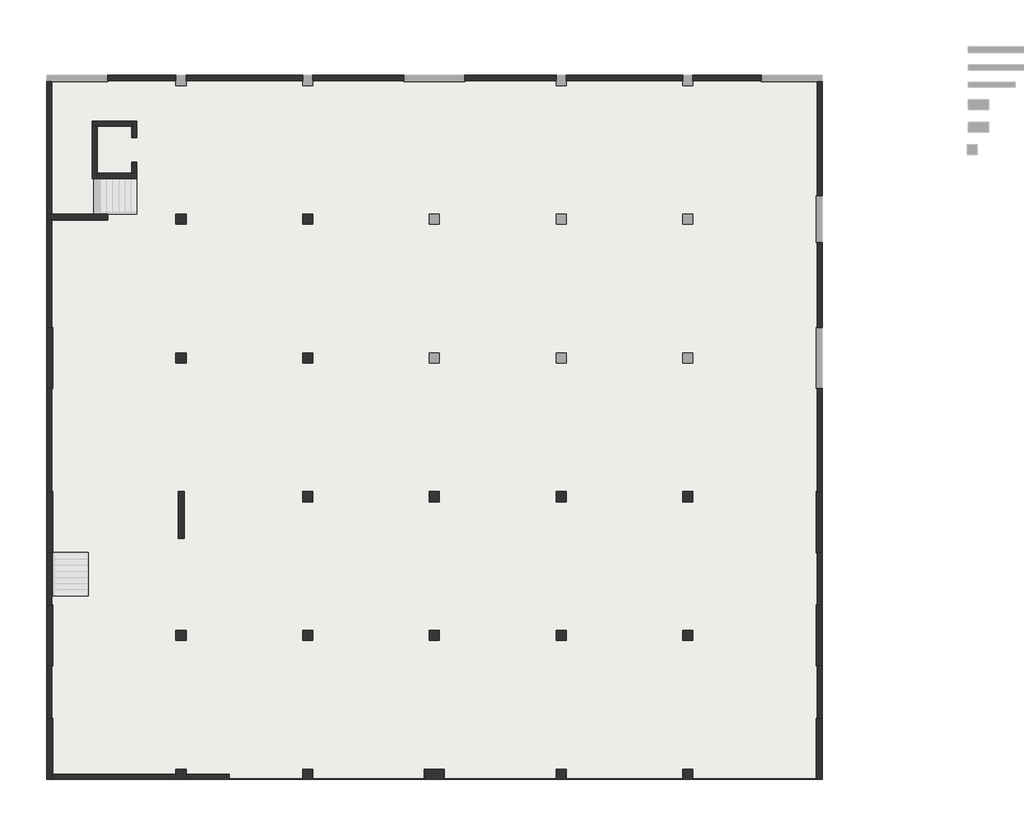
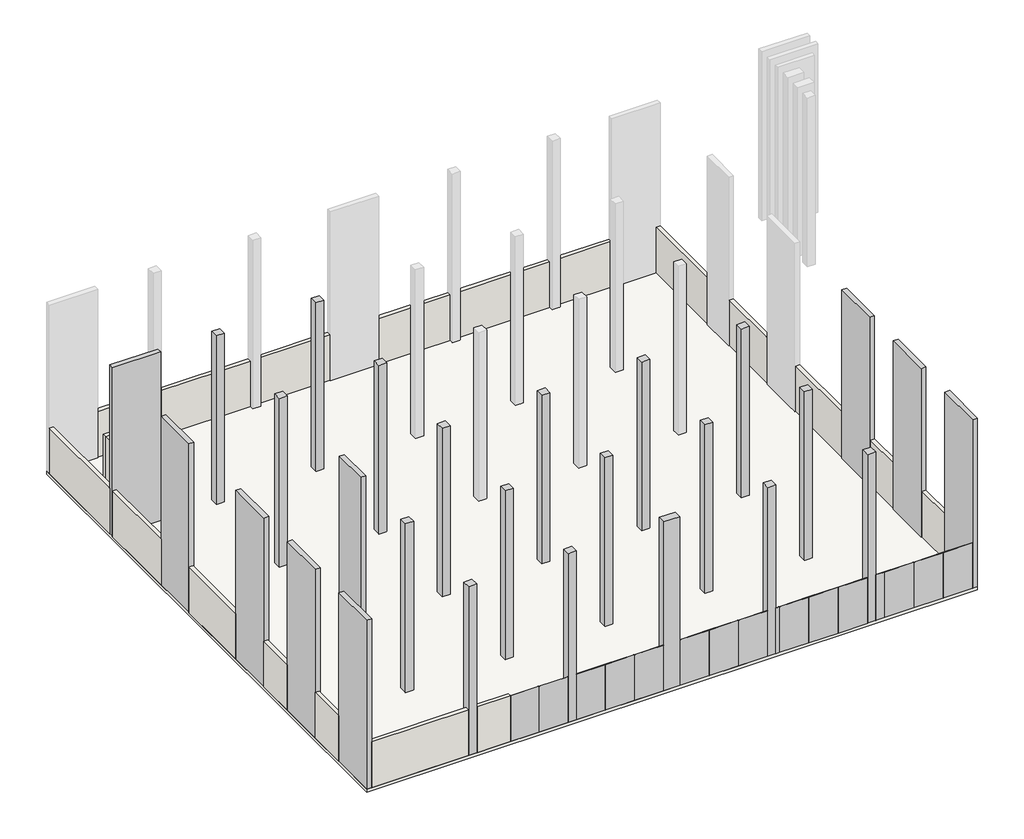
# One storey, part 1 of 2: 27 columns, 23 walls, 16 plates, 1 slab.
"""IFC4 building model written with IfcOpenShell, lengths in millimetres."""

import ifcopenshell
import ifcopenshell.guid

model = None  # the IFC model being written
_history = None  # IfcOwnerHistory: only IFC2X3 demands one
_inside = {}  # id of a spatial element -> (the spatial element, [elements in it])
_under = {}  # id of a project, library or spatial element -> (it, [spatial elements below it])
_declared = {}  # id of a project -> (the project, [libraries it declares])
_typed = {}  # id of a type object -> (the type object, [elements of that type])
_made_of = {}  # id of a material, layer set ... -> (it, [elements and type objects made of it])


def new_model(schema):
    """Start an empty IFC model of exactly this schema.

    Asked for "IFC4X3", IfcOpenShell would pick the latest addendum, in which some entities
    have other attributes; the version numbers below select the first issue.
    IFC2X3 requires an IfcOwnerHistory on every rooted entity: one is made here for all.
    """
    global model, _history
    if schema == "IFC4X3":
        model = ifcopenshell.file(schema_version=(4, 3, 0, 0))
    else:
        model = ifcopenshell.file(schema=schema)
    _inside.clear()
    _under.clear()
    _declared.clear()
    _typed.clear()
    _made_of.clear()
    _history = None
    if model.schema == "IFC2X3":
        org = make("IfcOrganization", Name="unknown")
        user = make(
            "IfcPersonAndOrganization",
            ThePerson=make("IfcPerson", FamilyName="unknown"),
            TheOrganization=org,
        )
        app = make(
            "IfcApplication",
            ApplicationDeveloper=org,
            Version="unknown",
            ApplicationFullName="unknown",
            ApplicationIdentifier="unknown",
        )
        _history = make(
            "IfcOwnerHistory",
            OwningUser=user,
            OwningApplication=app,
            ChangeAction="ADDED",
            CreationDate=0,
        )
    return model


def make(cls, **values):
    """One entity of the class cls with the attributes given. An attribute that is None is left unset."""
    return model.create_entity(
        cls, **{name: value for name, value in values.items() if value is not None}
    )


def rooted(cls, **values):
    """An entity with a GlobalId (a new one), such as an element, a storey or a relation."""
    return make(cls, GlobalId=ifcopenshell.guid.new(), OwnerHistory=_history, **values)


def si_unit(unit_type, name, prefix=None):
    """IfcSIUnit, for example si_unit("LENGTHUNIT", "METRE", prefix="MILLI")."""
    return make("IfcSIUnit", UnitType=unit_type, Prefix=prefix, Name=name)


def assignment(units):
    """IfcUnitAssignment: the units of a project."""
    return None if units is None else make("IfcUnitAssignment", Units=units)


def point(xyz):
    """IfcCartesianPoint."""
    return None if xyz is None else make("IfcCartesianPoint", Coordinates=xyz)


def direction(xyz):
    """IfcDirection."""
    return None if xyz is None else make("IfcDirection", DirectionRatios=xyz)


def frame(location, z_axis=None, x_axis=None):
    """IfcAxis2Placement3D, a coordinate frame: its origin and axes. An axis left out is left unset."""
    return make(
        "IfcAxis2Placement3D",
        Location=point(location),
        Axis=direction(z_axis),
        RefDirection=direction(x_axis),
    )


def origin():
    """The frame at (0, 0, 0) with its axes left unset."""
    return frame((0.0, 0.0, 0.0))


def origin_with_axes():
    """The frame at (0, 0, 0) with the z axis (0, 0, 1) and the x axis (1, 0, 0) written out."""
    return frame((0.0, 0.0, 0.0), z_axis=(0.0, 0.0, 1.0), x_axis=(1.0, 0.0, 0.0))


def place(relative_to, where):
    """IfcLocalPlacement: puts the frame where relative to a parent placement (None: the world)."""
    return make(
        "IfcLocalPlacement", PlacementRelTo=relative_to, RelativePlacement=where
    )


def context(
    kind, dimensions, precision=None, world=None, true_north=None, identifier=None
):
    """IfcGeometricRepresentationContext, for example the 3D "Model" context."""
    return make(
        "IfcGeometricRepresentationContext",
        ContextIdentifier=identifier,
        ContextType=kind,
        CoordinateSpaceDimension=dimensions,
        Precision=precision,
        WorldCoordinateSystem=world,
        TrueNorth=true_north,
    )


def project(units=None, contexts=None):
    """IfcProject with its units and contexts."""
    return rooted(
        "IfcProject",
        Name="project",
        RepresentationContexts=contexts,
        UnitsInContext=assignment(units),
    )


def spatial(cls, under=None, at=None, **own):
    """A site, building, storey or space (cls), placed at a placement, below another one or the project."""
    s = rooted(cls, ObjectPlacement=at, **own)
    if under is not None:
        _under.setdefault(under.id(), (under, []))[1].append(s)
    return s


def polyline(points):
    """IfcPolyline through the points."""
    return make("IfcPolyline", Points=[point(p) for p in points])


def outline(outer, holes=None, kind="AREA"):
    """IfcArbitraryClosedProfileDef: a profile drawn as a closed curve; with holes, ...WithVoids."""
    if holes is None:
        return make("IfcArbitraryClosedProfileDef", ProfileType=kind, OuterCurve=outer)
    return make(
        "IfcArbitraryProfileDefWithVoids",
        ProfileType=kind,
        OuterCurve=outer,
        InnerCurves=holes,
    )


def extrude(swept, where, along, depth):
    """IfcExtrudedAreaSolid: the profile swept, set in the frame where, extruded along a direction by depth."""
    return make(
        "IfcExtrudedAreaSolid",
        SweptArea=swept,
        Position=where,
        ExtrudedDirection=direction(along),
        Depth=depth,
    )


def faces_of(points, faces, orient=None, outer=None):
    """IfcFace entities. A face is a list of loops; a loop is a list of indices into points, from 0.

    orient and outer hold one flag for each loop. By default every Orientation is true, the
    first loop of a face is its IfcFaceOuterBound and the others are IfcFaceBound.
    """
    made = []
    for i, loops in enumerate(faces):
        bounds = []
        for j, loop in enumerate(loops):
            is_outer = j == 0 if outer is None else outer[i][j]
            bounds.append(
                make(
                    "IfcFaceOuterBound" if is_outer else "IfcFaceBound",
                    Bound=make("IfcPolyLoop", Polygon=[points[k] for k in loop]),
                    Orientation=True if orient is None else orient[i][j],
                )
            )
        made.append(make("IfcFace", Bounds=bounds))
    return made


def faceted_brep(points, faces, orient=None, outer=None, voids=None):
    """IfcFacetedBrep: a solid bounded by flat faces; with voids (closed shells), ...WithVoids."""
    shared = [point(p) for p in points]
    hull = make("IfcClosedShell", CfsFaces=faces_of(shared, faces, orient, outer))
    if voids is None:
        return make("IfcFacetedBrep", Outer=hull)
    return make(
        "IfcFacetedBrepWithVoids",
        Outer=hull,
        Voids=[
            make(cls, CfsFaces=faces_of(shared, fs, o, b)) for cls, fs, o, b in voids
        ],
    )


def shape(context_of_items, identifier, shape_type, items):
    """IfcShapeRepresentation: the items that make up one representation, for example the "Body"."""
    return make(
        "IfcShapeRepresentation",
        ContextOfItems=context_of_items,
        RepresentationIdentifier=identifier,
        RepresentationType=shape_type,
        Items=items,
    )


def source(mapping_origin, context_of_items, identifier, shape_type, items):
    """IfcRepresentationMap: a shape defined once, which mapped items show again and again."""
    return make(
        "IfcRepresentationMap",
        MappingOrigin=mapping_origin,
        MappedRepresentation=shape(context_of_items, identifier, shape_type, items),
    )


def transform(
    local_origin,
    x_axis=None,
    y_axis=None,
    z_axis=None,
    scale=None,
    scale2=None,
    scale3=None,
    uniform=True,
):
    """IfcCartesianTransformationOperator3D, or its non-uniform kind. x_axis, y_axis, z_axis: its Axis1, 2, 3."""
    if uniform:
        return make(
            "IfcCartesianTransformationOperator3D",
            Axis1=direction(x_axis),
            Axis2=direction(y_axis),
            LocalOrigin=point(local_origin),
            Scale=scale,
            Axis3=direction(z_axis),
        )
    return make(
        "IfcCartesianTransformationOperator3DnonUniform",
        Axis1=direction(x_axis),
        Axis2=direction(y_axis),
        LocalOrigin=point(local_origin),
        Scale=scale,
        Axis3=direction(z_axis),
        Scale2=scale2,
        Scale3=scale3,
    )


def mapped(mapping_source, mapping_target):
    """IfcMappedItem: shows the shape of a source again, moved by a transform."""
    return make(
        "IfcMappedItem", MappingSource=mapping_source, MappingTarget=mapping_target
    )


def made_of(thing, what):
    """Note that an element or type object is made of a material, layer set ...; save() writes the relation."""
    if what is not None:
        _made_of.setdefault(what.id(), (what, []))[1].append(thing)
    return thing


def element(
    cls,
    number,
    at=None,
    inside=None,
    cuts=None,
    type_object=None,
    material=None,
    context=None,
    identifier="Body",
    shape_type=None,
    held_by="IfcProductDefinitionShape",
    body=None,
    shapes=None,
    **own,
):
    """One element of the class cls, such as IfcWall. Its Tag is "e" and its number.

    at: its placement. inside: the storey or other place that contains it. cuts: it is an
    opening in that element (IfcRelVoidsElement). A single representation is given by context,
    identifier, shape_type and body (its items); several are given by shapes. held_by: the class
    of the entity that holds the representations. save() writes the other relations.
    """
    e = rooted(cls, Tag="e%d" % number, ObjectPlacement=at, **own)
    if body is not None:
        shapes = [shape(context, identifier, shape_type, body)]
    if shapes is not None:
        e.Representation = make(held_by, Representations=shapes)
    if inside is not None:
        _inside.setdefault(inside.id(), (inside, []))[1].append(e)
    if cuts is not None:
        rooted(
            "IfcRelVoidsElement", RelatingBuildingElement=cuts, RelatedOpeningElement=e
        )
    if type_object is not None:
        _typed.setdefault(type_object.id(), (type_object, []))[1].append(e)
    return made_of(e, material)


def aggregate(whole, parts):
    """IfcRelAggregates: a whole, such as a stair, and the parts it consists of."""
    return rooted("IfcRelAggregates", RelatingObject=whole, RelatedObjects=parts)


def save(model, path):
    """Write the relations noted so far, then the file.

    IfcRelAggregates (storeys below a building ...), IfcRelContainedInSpatialStructure (elements
    in a storey), IfcRelDefinesByType, IfcRelAssociatesMaterial and IfcRelDeclares: one each for
    every whole, place, type object, material and project.
    """
    for whole, parts in _under.values():
        aggregate(whole, parts)
    for where, things in _inside.values():
        rooted(
            "IfcRelContainedInSpatialStructure",
            RelatedElements=things,
            RelatingStructure=where,
        )
    for kind, things in _typed.values():
        rooted("IfcRelDefinesByType", RelatedObjects=things, RelatingType=kind)
    for what, things in _made_of.values():
        rooted("IfcRelAssociatesMaterial", RelatedObjects=things, RelatingMaterial=what)
    for by, libraries in _declared.values():
        rooted("IfcRelDeclares", RelatingContext=by, RelatedDefinitions=libraries)
    model.write(path)


def m_rectangular_column_100x50_89a3459c(model_context):
    return source(origin(), model_context, "Body", "SweptSolid", [
        extrude(outline(polyline([(500.0, 250.0), (500.0, -250.0), (-500.0, -250.0), (-500.0, 250.0), (500.0, 250.0)])), frame((0.0, 0.0, -3200.0), z_axis=(0.0, 0.0, 1.0), x_axis=(1.0, 0.0, 0.0)), (0.0, 0.0, 1.0), 11100.0),
    ])


def m_rectangular_column_230x30_624f9335(model_context):
    return source(origin(), model_context, "Body", "SweptSolid", [
        extrude(outline(polyline([(1150.0, 150.0), (1150.0, -150.0), (-1150.0, -150.0), (-1150.0, 150.0), (1150.0, 150.0)])), frame((0.0, 0.0, -3200.0), z_axis=(0.0, 0.0, 1.0), x_axis=(1.0, 0.0, 0.0)), (0.0, 0.0, 1.0), 11100.0),
    ])


def m_rectangular_column_300x30_b7aa0491(model_context):
    return source(origin(), model_context, "Body", "SweptSolid", [
        extrude(outline(polyline([(1500.0, 150.0), (1500.0, -150.0), (-1500.0, -150.0), (-1500.0, 150.0), (1500.0, 150.0)])), frame((0.0, 0.0, -3200.0), z_axis=(0.0, 0.0, 1.0), x_axis=(1.0, 0.0, 0.0)), (0.0, 0.0, 1.0), 11100.0),
    ])


def m_rectangular_column_300x30_baf48ca4(model_context):
    return source(origin(), model_context, "Body", "SweptSolid", [
        extrude(outline(polyline([(1500.0, -150.0), (-1500.0, -150.0), (-1500.0, 150.0), (1500.0, 150.0), (1500.0, -150.0)])), frame((0.0, 0.0, -3200.0), z_axis=(0.0, 0.0, 1.0), x_axis=(1.0, 0.0, 0.0)), (0.0, 0.0, 1.0), 11100.0),
    ])


def m_rectangular_column_50x50_3a95f3c9(model_context):
    return source(origin(), model_context, "Body", "SweptSolid", [
        extrude(outline(polyline([(250.0, 250.0), (250.0, -250.0), (-250.0, -250.0), (-250.0, 250.0), (250.0, 250.0)])), frame((0.0, 0.0, -3200.0), z_axis=(0.0, 0.0, 1.0), x_axis=(1.0, 0.0, 0.0)), (0.0, 0.0, 1.0), 11100.0),
    ])


def system_panel_glazed_1b9f2f65(model_context):
    return source(origin(), model_context, "Body", "SweptSolid", [
        extrude(outline(polyline([(915.0000002, 24.5), (-915.0000002, 24.5), (-915.0000002, 49.5), (915.0000002, 49.5), (915.0000002, 24.5)])), origin_with_axes(), (0.0, 0.0, 1.0), 3000.0),
    ])


def system_panel_glazed_a36a1bad(model_context):
    return source(origin(), model_context, "Body", "SweptSolid", [
        extrude(outline(polyline([(274.9999998, 24.5), (-274.9999998, 24.5), (-274.9999998, 49.5), (274.9999998, 49.5), (274.9999998, 24.5)])), origin_with_axes(), (0.0, 0.0, 1.0), 3000.0),
    ])


def system_panel_glazed_34b19285(model_context):
    return source(origin(), model_context, "Body", "SweptSolid", [
        extrude(outline(polyline([(104.9999998, 24.5), (-104.9999998, 24.5), (-104.9999998, 49.5), (104.9999998, 49.5), (104.9999998, 24.5)])), origin_with_axes(), (0.0, 0.0, 1.0), 3000.0),
    ])


def system_panel_glazed_557d3a43(model_context):
    return source(origin(), model_context, "Body", "SweptSolid", [
        extrude(outline(polyline([(904.9999998, 24.5), (-904.9999998, 24.5), (-904.9999998, 49.5), (904.9999998, 49.5), (904.9999998, 24.5)])), origin_with_axes(), (0.0, 0.0, 1.0), 3000.0),
    ])


def system_panel_glazed_35b321d4(model_context):
    return source(origin(), model_context, "Body", "SweptSolid", [
        extrude(outline(polyline([(894.9999998, 24.5), (-894.9999998, 24.5), (-894.9999998, 49.5), (894.9999998, 49.5), (894.9999998, 24.5)])), origin_with_axes(), (0.0, 0.0, 1.0), 3000.0),
    ])


def system_panel_glazed_d48c6481(model_context):
    return source(origin(), model_context, "Body", "SweptSolid", [
        extrude(outline(polyline([(879.9999998, 24.5), (-879.9999998, 24.5), (-879.9999998, 49.5), (879.9999998, 49.5), (879.9999998, 24.5)])), origin_with_axes(), (0.0, 0.0, 1.0), 3000.0),
    ])


model = new_model("IFC4")

# Units and contexts
model_context = context("Model", 3, world=origin())
ifc_project = project(units=[si_unit("LENGTHUNIT", "METRE", prefix="MILLI")], contexts=[model_context])

# Site, building, storey
site = spatial("IfcSite", under=ifc_project)
building = spatial("IfcBuilding", under=site)
storey = spatial("IfcBuildingStorey", under=building, Name="Bodrumi", Elevation=-3200.0)

# Columns
placement = place(None, origin())
m_rectangular_column_100x50_shape = m_rectangular_column_100x50_89a3459c(model_context)
element("IfcColumn", 1, ObjectType="M_Rectangular Column : 100x50", at=placement, inside=storey, context=model_context, shape_type="MappedRepresentation", body=[
    mapped(m_rectangular_column_100x50_shape, transform((1115.581911, -16469.3231037, 0.0), x_axis=(1.0, 0.0, 0.0), y_axis=(0.0, 1.0, 0.0), z_axis=(0.0, 0.0, 1.0))),
])
m_rectangular_column_230x30_shape = m_rectangular_column_230x30_624f9335(model_context)
element("IfcColumn", 2, ObjectType="M_Rectangular Column : 230x30", at=placement, inside=storey, context=model_context, shape_type="MappedRepresentation", body=[
    mapped(m_rectangular_column_230x30_shape, transform((-11284.418089, -3769.3231037, 0.0), x_axis=(0.0, 1.0, 0.0), y_axis=(-1.0, 0.0, 0.0), z_axis=(0.0, 0.0, 1.0))),
])
element("IfcColumn", 3, ObjectType="M_Rectangular Column : 300x30", at=placement, inside=storey, context=model_context, shape_type="SweptSolid", body=[
    extrude(outline(polyline([(-14874.418089, 10980.6768963), (-14874.418089, 10680.6768963), (-17874.418089, 10680.6768963), (-17874.418089, 10980.6768963), (-14874.418089, 10980.6768963)])), frame((0.0, 0.0, -3200.0), z_axis=(0.0, 0.0, 1.0), x_axis=(1.0, 0.0, 0.0)), (0.0, 0.0, 1.0), 11100.0),
])
m_rectangular_column_300x30_shape = m_rectangular_column_300x30_b7aa0491(model_context)
element("IfcColumn", 4, ObjectType="M_Rectangular Column : 300x30", at=placement, inside=storey, context=model_context, shape_type="MappedRepresentation", body=[
    mapped(m_rectangular_column_300x30_shape, transform((-17724.418089, -15219.3231037, 0.0), x_axis=(0.0, 1.0, 0.0), y_axis=(-1.0, 0.0, 0.0), z_axis=(0.0, 0.0, 1.0))),
])
element("IfcColumn", 5, ObjectType="M_Rectangular Column : 300x30", at=placement, inside=storey, context=model_context, shape_type="MappedRepresentation", body=[
    mapped(m_rectangular_column_300x30_shape, transform((19975.581911, -15219.3231037, 0.0), x_axis=(0.0, 1.0, 0.0), y_axis=(-1.0, 0.0, 0.0), z_axis=(0.0, 0.0, 1.0))),
])
element("IfcColumn", 6, ObjectType="M_Rectangular Column : 300x30", at=placement, inside=storey, context=model_context, shape_type="MappedRepresentation", body=[
    mapped(m_rectangular_column_300x30_shape, transform((19975.581911, -4119.3231037, 0.0), x_axis=(0.0, 1.0, 0.0), y_axis=(-1.0, 0.0, 0.0), z_axis=(0.0, 0.0, 1.0))),
])
element("IfcColumn", 7, ObjectType="M_Rectangular Column : 300x30", at=placement, inside=storey, context=model_context, shape_type="MappedRepresentation", body=[
    mapped(m_rectangular_column_300x30_shape, transform((19975.581911, -9669.3231037, 0.0), x_axis=(0.0, 1.0, 0.0), y_axis=(-1.0, 0.0, 0.0), z_axis=(0.0, 0.0, 1.0))),
])
m_rectangular_column_300x30_2_shape = m_rectangular_column_300x30_baf48ca4(model_context)
element("IfcColumn", 8, ObjectType="M_Rectangular Column : 300x30", at=placement, inside=storey, context=model_context, shape_type="MappedRepresentation", body=[
    mapped(m_rectangular_column_300x30_2_shape, transform((-17724.418089, 3930.6768963, 0.0), x_axis=(0.0, 1.0, 0.0), y_axis=(-1.0, 0.0, 0.0), z_axis=(0.0, 0.0, 1.0))),
])
element("IfcColumn", 9, ObjectType="M_Rectangular Column : 300x30", at=placement, inside=storey, context=model_context, shape_type="MappedRepresentation", body=[
    mapped(m_rectangular_column_300x30_2_shape, transform((-17724.418089, -4119.3231037, 0.0), x_axis=(0.0, 1.0, 0.0), y_axis=(-1.0, 0.0, 0.0), z_axis=(0.0, 0.0, 1.0))),
])
element("IfcColumn", 10, ObjectType="M_Rectangular Column : 300x30", at=placement, inside=storey, context=model_context, shape_type="MappedRepresentation", body=[
    mapped(m_rectangular_column_300x30_2_shape, transform((-17724.418089, -9669.3231037, 0.0), x_axis=(0.0, 1.0, 0.0), y_axis=(-1.0, 0.0, 0.0), z_axis=(0.0, 0.0, 1.0))),
])
m_rectangular_column_50x50_shape = m_rectangular_column_50x50_3a95f3c9(model_context)
element("IfcColumn", 11, ObjectType="M_Rectangular Column : 50x50", at=placement, inside=storey, context=model_context, shape_type="MappedRepresentation", body=[
    mapped(m_rectangular_column_50x50_shape, transform((-11284.418089, 10730.6768963, 0.0), x_axis=(1.0, 0.0, 0.0), y_axis=(0.0, 1.0, 0.0), z_axis=(0.0, 0.0, 1.0))),
])
element("IfcColumn", 12, ObjectType="M_Rectangular Column : 50x50", at=placement, inside=storey, context=model_context, shape_type="MappedRepresentation", body=[
    mapped(m_rectangular_column_50x50_shape, transform((-5084.418089, 10730.6768963, 0.0), x_axis=(1.0, 0.0, 0.0), y_axis=(0.0, 1.0, 0.0), z_axis=(0.0, 0.0, 1.0))),
])
element("IfcColumn", 13, ObjectType="M_Rectangular Column : 50x50", at=placement, inside=storey, context=model_context, shape_type="MappedRepresentation", body=[
    mapped(m_rectangular_column_50x50_shape, transform((-11284.418089, 3930.6768963, 0.0), x_axis=(1.0, 0.0, 0.0), y_axis=(0.0, 1.0, 0.0), z_axis=(0.0, 0.0, 1.0))),
])
element("IfcColumn", 14, ObjectType="M_Rectangular Column : 50x50", at=placement, inside=storey, context=model_context, shape_type="MappedRepresentation", body=[
    mapped(m_rectangular_column_50x50_shape, transform((-5084.418089, 3930.6768963, 0.0), x_axis=(1.0, 0.0, 0.0), y_axis=(0.0, 1.0, 0.0), z_axis=(0.0, 0.0, 1.0))),
])
element("IfcColumn", 15, ObjectType="M_Rectangular Column : 50x50", at=placement, inside=storey, context=model_context, shape_type="MappedRepresentation", body=[
    mapped(m_rectangular_column_50x50_shape, transform((13535.581911, -2869.3231037, 0.0), x_axis=(1.0, 0.0, 0.0), y_axis=(0.0, 1.0, 0.0), z_axis=(0.0, 0.0, 1.0))),
])
element("IfcColumn", 16, ObjectType="M_Rectangular Column : 50x50", at=placement, inside=storey, context=model_context, shape_type="MappedRepresentation", body=[
    mapped(m_rectangular_column_50x50_shape, transform((-5084.418089, -2869.3231037, 0.0), x_axis=(1.0, 0.0, 0.0), y_axis=(0.0, 1.0, 0.0), z_axis=(0.0, 0.0, 1.0))),
])
element("IfcColumn", 17, ObjectType="M_Rectangular Column : 50x50", at=placement, inside=storey, context=model_context, shape_type="MappedRepresentation", body=[
    mapped(m_rectangular_column_50x50_shape, transform((1115.581911, -2869.3231037, 0.0), x_axis=(1.0, 0.0, 0.0), y_axis=(0.0, 1.0, 0.0), z_axis=(0.0, 0.0, 1.0))),
])
element("IfcColumn", 18, ObjectType="M_Rectangular Column : 50x50", at=placement, inside=storey, context=model_context, shape_type="MappedRepresentation", body=[
    mapped(m_rectangular_column_50x50_shape, transform((7335.581911, -2869.3231037, 0.0), x_axis=(1.0, 0.0, 0.0), y_axis=(0.0, 1.0, 0.0), z_axis=(0.0, 0.0, 1.0))),
])
element("IfcColumn", 19, ObjectType="M_Rectangular Column : 50x50", at=placement, inside=storey, context=model_context, shape_type="MappedRepresentation", body=[
    mapped(m_rectangular_column_50x50_shape, transform((13535.581911, -9669.3231037, 0.0), x_axis=(1.0, 0.0, 0.0), y_axis=(0.0, 1.0, 0.0), z_axis=(0.0, 0.0, 1.0))),
])
element("IfcColumn", 20, ObjectType="M_Rectangular Column : 50x50", at=placement, inside=storey, context=model_context, shape_type="MappedRepresentation", body=[
    mapped(m_rectangular_column_50x50_shape, transform((-11284.418089, -9669.3231037, 0.0), x_axis=(1.0, 0.0, 0.0), y_axis=(0.0, 1.0, 0.0), z_axis=(0.0, 0.0, 1.0))),
])
element("IfcColumn", 21, ObjectType="M_Rectangular Column : 50x50", at=placement, inside=storey, context=model_context, shape_type="MappedRepresentation", body=[
    mapped(m_rectangular_column_50x50_shape, transform((-5084.418089, -9669.3231037, 0.0), x_axis=(1.0, 0.0, 0.0), y_axis=(0.0, 1.0, 0.0), z_axis=(0.0, 0.0, 1.0))),
])
element("IfcColumn", 22, ObjectType="M_Rectangular Column : 50x50", at=placement, inside=storey, context=model_context, shape_type="MappedRepresentation", body=[
    mapped(m_rectangular_column_50x50_shape, transform((1115.581911, -9669.3231037, 0.0), x_axis=(1.0, 0.0, 0.0), y_axis=(0.0, 1.0, 0.0), z_axis=(0.0, 0.0, 1.0))),
])
element("IfcColumn", 23, ObjectType="M_Rectangular Column : 50x50", at=placement, inside=storey, context=model_context, shape_type="MappedRepresentation", body=[
    mapped(m_rectangular_column_50x50_shape, transform((7335.581911, -9669.3231037, 0.0), x_axis=(1.0, 0.0, 0.0), y_axis=(0.0, 1.0, 0.0), z_axis=(0.0, 0.0, 1.0))),
])
element("IfcColumn", 24, ObjectType="M_Rectangular Column : 50x50", at=placement, inside=storey, context=model_context, shape_type="MappedRepresentation", body=[
    mapped(m_rectangular_column_50x50_shape, transform((13535.581911, -16469.3231037, 0.0), x_axis=(1.0, 0.0, 0.0), y_axis=(0.0, 1.0, 0.0), z_axis=(0.0, 0.0, 1.0))),
])
element("IfcColumn", 25, ObjectType="M_Rectangular Column : 50x50", at=placement, inside=storey, context=model_context, shape_type="MappedRepresentation", body=[
    mapped(m_rectangular_column_50x50_shape, transform((-11284.418089, -16469.3231037, 0.0), x_axis=(1.0, 0.0, 0.0), y_axis=(0.0, 1.0, 0.0), z_axis=(0.0, 0.0, 1.0))),
])
element("IfcColumn", 26, ObjectType="M_Rectangular Column : 50x50", at=placement, inside=storey, context=model_context, shape_type="MappedRepresentation", body=[
    mapped(m_rectangular_column_50x50_shape, transform((-5084.418089, -16469.3231037, 0.0), x_axis=(1.0, 0.0, 0.0), y_axis=(0.0, 1.0, 0.0), z_axis=(0.0, 0.0, 1.0))),
])
element("IfcColumn", 27, ObjectType="M_Rectangular Column : 50x50", at=placement, inside=storey, context=model_context, shape_type="MappedRepresentation", body=[
    mapped(m_rectangular_column_50x50_shape, transform((7335.581911, -16469.3231037, 0.0), x_axis=(1.0, 0.0, 0.0), y_axis=(0.0, 1.0, 0.0), z_axis=(0.0, 0.0, 1.0))),
])

# Plates
system_panel_glazed_shape = system_panel_glazed_1b9f2f65(model_context)
element("IfcPlate", 28, ObjectType="System Panel : Glazed", at=placement, inside=storey, context=model_context, shape_type="MappedRepresentation", body=[
    mapped(system_panel_glazed_shape, transform((18910.5819109, -16669.3231037, -3200.0), x_axis=(-1.0, 0.0, 0.0), y_axis=(0.0, -1.0, 0.0), z_axis=(0.0, 0.0, 1.0))),
])
element("IfcPlate", 29, ObjectType="System Panel : Glazed", at=placement, inside=storey, context=model_context, shape_type="MappedRepresentation", body=[
    mapped(system_panel_glazed_shape, transform((17080.5819107, -16669.3231037, -3200.0), x_axis=(-1.0, 0.0, 0.0), y_axis=(0.0, -1.0, 0.0), z_axis=(0.0, 0.0, 1.0))),
])
element("IfcPlate", 30, ObjectType="System Panel : Glazed", at=placement, inside=storey, context=model_context, shape_type="MappedRepresentation", body=[
    mapped(system_panel_glazed_shape, transform((15250.5819107, -16669.3231037, -3200.0), x_axis=(-1.0, 0.0, 0.0), y_axis=(0.0, -1.0, 0.0), z_axis=(0.0, 0.0, 1.0))),
])
element("IfcPlate", 31, ObjectType="System Panel : Glazed", at=placement, inside=storey, context=model_context, shape_type="MappedRepresentation", body=[
    mapped(system_panel_glazed_shape, transform((12370.5819109, -16669.9481037, -3200.0), x_axis=(-1.0, 0.0, 0.0), y_axis=(0.0, -1.0, 0.0), z_axis=(0.0, 0.0, 1.0))),
])
element("IfcPlate", 32, ObjectType="System Panel : Glazed", at=placement, inside=storey, context=model_context, shape_type="MappedRepresentation", body=[
    mapped(system_panel_glazed_shape, transform((10540.5819107, -16669.9481037, -3200.0), x_axis=(-1.0, 0.0, 0.0), y_axis=(0.0, -1.0, 0.0), z_axis=(0.0, 0.0, 1.0))),
])
element("IfcPlate", 33, ObjectType="System Panel : Glazed", at=placement, inside=storey, context=model_context, shape_type="MappedRepresentation", body=[
    mapped(system_panel_glazed_shape, transform((8710.5819107, -16669.9481037, -3200.0), x_axis=(-1.0, 0.0, 0.0), y_axis=(0.0, -1.0, 0.0), z_axis=(0.0, 0.0, 1.0))),
])
element("IfcPlate", 34, ObjectType="System Panel : Glazed", at=placement, inside=storey, context=model_context, shape_type="MappedRepresentation", body=[
    mapped(system_panel_glazed_shape, transform((6170.5819109, -16669.3231037, -3200.0), x_axis=(-1.0, 0.0, 0.0), y_axis=(0.0, -1.0, 0.0), z_axis=(0.0, 0.0, 1.0))),
])
element("IfcPlate", 35, ObjectType="System Panel : Glazed", at=placement, inside=storey, context=model_context, shape_type="MappedRepresentation", body=[
    mapped(system_panel_glazed_shape, transform((4340.5819107, -16669.3231037, -3200.0), x_axis=(-1.0, 0.0, 0.0), y_axis=(0.0, -1.0, 0.0), z_axis=(0.0, 0.0, 1.0))),
])
element("IfcPlate", 36, ObjectType="System Panel : Glazed", at=placement, inside=storey, context=model_context, shape_type="MappedRepresentation", body=[
    mapped(system_panel_glazed_shape, transform((-299.4180891, -16669.3231037, -3200.0), x_axis=(-1.0, 0.0, 0.0), y_axis=(0.0, -1.0, 0.0), z_axis=(0.0, 0.0, 1.0))),
])
element("IfcPlate", 37, ObjectType="System Panel : Glazed", at=placement, inside=storey, context=model_context, shape_type="MappedRepresentation", body=[
    mapped(system_panel_glazed_shape, transform((-2129.4180893, -16669.3231037, -3200.0), x_axis=(-1.0, 0.0, 0.0), y_axis=(0.0, -1.0, 0.0), z_axis=(0.0, 0.0, 1.0))),
])
element("IfcPlate", 38, ObjectType="System Panel : Glazed", at=placement, inside=storey, context=model_context, shape_type="MappedRepresentation", body=[
    mapped(system_panel_glazed_shape, transform((-6249.4180891, -16669.3231037, -3200.0), x_axis=(-1.0, 0.0, 0.0), y_axis=(0.0, -1.0, 0.0), z_axis=(0.0, 0.0, 1.0))),
])
system_panel_glazed_2_shape = system_panel_glazed_a36a1bad(model_context)
element("IfcPlate", 39, ObjectType="System Panel : Glazed", at=placement, inside=storey, context=model_context, shape_type="MappedRepresentation", body=[
    mapped(system_panel_glazed_2_shape, transform((14060.5819109, -16669.3231037, -3200.0), x_axis=(-1.0, 0.0, 0.0), y_axis=(0.0, -1.0, 0.0), z_axis=(0.0, 0.0, 1.0))),
])
system_panel_glazed_3_shape = system_panel_glazed_34b19285(model_context)
element("IfcPlate", 40, ObjectType="System Panel : Glazed", at=placement, inside=storey, context=model_context, shape_type="MappedRepresentation", body=[
    mapped(system_panel_glazed_3_shape, transform((7690.5819109, -16669.9481037, -3200.0), x_axis=(-1.0, 0.0, 0.0), y_axis=(0.0, -1.0, 0.0), z_axis=(0.0, 0.0, 1.0))),
])
system_panel_glazed_4_shape = system_panel_glazed_557d3a43(model_context)
element("IfcPlate", 41, ObjectType="System Panel : Glazed", at=placement, inside=storey, context=model_context, shape_type="MappedRepresentation", body=[
    mapped(system_panel_glazed_4_shape, transform((2520.5819109, -16669.3231037, -3200.0), x_axis=(-1.0, 0.0, 0.0), y_axis=(0.0, -1.0, 0.0), z_axis=(0.0, 0.0, 1.0))),
])
system_panel_glazed_5_shape = system_panel_glazed_35b321d4(model_context)
element("IfcPlate", 42, ObjectType="System Panel : Glazed", at=placement, inside=storey, context=model_context, shape_type="MappedRepresentation", body=[
    mapped(system_panel_glazed_5_shape, transform((-3939.4180891, -16669.3231037, -3200.0), x_axis=(-1.0, 0.0, 0.0), y_axis=(0.0, -1.0, 0.0), z_axis=(0.0, 0.0, 1.0))),
])
system_panel_glazed_6_shape = system_panel_glazed_d48c6481(model_context)
element("IfcPlate", 43, ObjectType="System Panel : Glazed", at=placement, inside=storey, context=model_context, shape_type="MappedRepresentation", body=[
    mapped(system_panel_glazed_6_shape, transform((-8044.4180891, -16669.3231037, -3200.0), x_axis=(-1.0, 0.0, 0.0), y_axis=(0.0, -1.0, 0.0), z_axis=(0.0, 0.0, 1.0))),
])

# Slab
element("IfcSlab", 44, ObjectType="Generic 20", at=placement, inside=storey, context=model_context, shape_type="SweptSolid", body=[
    extrude(outline(polyline([(20125.581911, 17780.6768963), (20125.581911, -16719.3231037), (-17874.418089, -16719.3231037), (-17874.418089, 17780.6768963), (20125.581911, 17780.6768963)])), frame((0.0, 0.0, -3400.0), z_axis=(0.0, 0.0, 1.0), x_axis=(1.0, 0.0, 0.0)), (0.0, 0.0, 1.0), 200.0),
])

# Walls
element("IfcWall", 45, ObjectType="lifti", at=placement, inside=storey, context=model_context, shape_type="Brep", body=[
    faceted_brep([(-15644.418089, 15280.6768963, -3200.0), (-15394.418089, 15280.6768963, -3200.0), (-13694.418089, 15280.6768963, -3200.0), (-13694.418089, 15280.6768963, -200.0), (-15394.418089, 15280.6768963, -200.0), (-15644.418089, 15280.6768963, -200.0), (-15644.418089, 15530.6768963, -3200.0), (-15644.418089, 15530.6768963, -200.0), (-13694.418089, 15530.6768963, -200.0), (-13694.418089, 15530.6768963, -3200.0)], [[[0, 1, 2, 3, 4, 5]], [[6, 7, 8, 9]], [[2, 1, 0, 6, 9]], [[5, 4, 3, 8, 7]], [[0, 5, 7, 6]], [[3, 2, 9, 8]]]),
])
element("IfcWall", 46, ObjectType="lifti", at=placement, inside=storey, context=model_context, shape_type="Brep", body=[
    faceted_brep([(-15394.418089, 12730.6768963, -3200.0), (-15394.418089, 12980.6768963, -3200.0), (-15394.418089, 15280.6768963, -3200.0), (-15394.418089, 15280.6768963, -200.0), (-15394.418089, 12980.6768963, -200.0), (-15394.418089, 12730.6768963, -200.0), (-15644.418089, 12730.6768963, -3200.0), (-15644.418089, 12730.6768963, -200.0), (-15644.418089, 15280.6768963, -200.0), (-15644.418089, 15280.6768963, -3200.0)], [[[0, 1, 2, 3, 4, 5]], [[6, 7, 8, 9]], [[2, 1, 0, 6, 9]], [[5, 4, 3, 8, 7]], [[0, 5, 7, 6]], [[3, 2, 9, 8]]]),
])
element("IfcWall", 47, ObjectType="lifti", at=placement, inside=storey, context=model_context, shape_type="Brep", body=[
    faceted_brep([(-13444.418089, 12980.6768963, -3200.0), (-13694.418089, 12980.6768963, -3200.0), (-15394.418089, 12980.6768963, -3200.0), (-15394.418089, 12980.6768963, -200.0), (-13694.418089, 12980.6768963, -200.0), (-13444.418089, 12980.6768963, -200.0), (-13444.418089, 12730.6768963, -3200.0), (-13444.418089, 12730.6768963, -200.0), (-15394.418089, 12730.6768963, -200.0), (-15394.418089, 12730.6768963, -3200.0)], [[[0, 1, 2, 3, 4, 5]], [[6, 7, 8, 9]], [[2, 1, 0, 6, 9]], [[5, 4, 3, 8, 7]], [[0, 5, 7, 6]], [[3, 2, 9, 8]]]),
])
element("IfcWall", 48, ObjectType="lifti", at=placement, inside=storey, context=model_context, shape_type="Brep", body=[
    faceted_brep([(-13694.418089, 15530.6768963, -3200.0), (-13694.418089, 15280.6768963, -3200.0), (-13694.418089, 14730.6768963, -3200.0), (-13694.418089, 14730.6768963, -200.0), (-13694.418089, 15280.6768963, -200.0), (-13694.418089, 15530.6768963, -200.0), (-13444.418089, 15530.6768963, -3200.0), (-13444.418089, 15530.6768963, -200.0), (-13444.418089, 14730.6768963, -200.0), (-13444.418089, 14730.6768963, -3200.0)], [[[0, 1, 2, 3, 4, 5]], [[6, 7, 8, 9]], [[2, 1, 0, 6, 9]], [[3, 2, 9, 8]], [[5, 4, 3, 8, 7]], [[0, 5, 7, 6]]]),
])
element("IfcWall", 49, ObjectType="lifti", at=placement, inside=storey, context=model_context, shape_type="SweptSolid", body=[
    extrude(outline(polyline([(-13694.418089, 12980.6768963), (-13694.418089, 13530.6768963), (-13444.418089, 13530.6768963), (-13444.418089, 12980.6768963), (-13694.418089, 12980.6768963)])), frame((0.0, 0.0, -3200.0), z_axis=(0.0, 0.0, 1.0), x_axis=(1.0, 0.0, 0.0)), (0.0, 0.0, 1.0), 3000.0),
])
element("IfcWall", 50, ObjectType="Generic - 250", at=placement, inside=storey, context=model_context, shape_type="SweptSolid", body=[
    extrude(outline(polyline([(-17874.418089, 10980.6768963), (-17874.418089, 17480.6768963), (-17624.418089, 17480.6768963), (-17624.418089, 10980.6768963), (-17874.418089, 10980.6768963)])), frame((0.0, 0.0, -3200.0), z_axis=(0.0, 0.0, 1.0), x_axis=(1.0, 0.0, 0.0)), (0.0, 0.0, 1.0), 3000.0),
])
element("IfcWall", 51, ObjectType="Generic - 250", at=placement, inside=storey, context=model_context, shape_type="SweptSolid", body=[
    extrude(outline(polyline([(-11534.418089, 17530.6768963), (-14874.418089, 17530.6768963), (-14874.418089, 17780.6768963), (-11534.418089, 17780.6768963), (-11534.418089, 17530.6768963)])), frame((0.0, 0.0, -3200.0), z_axis=(0.0, 0.0, 1.0), x_axis=(1.0, 0.0, 0.0)), (0.0, 0.0, 1.0), 3000.0),
])
element("IfcWall", 52, ObjectType="Generic - 250", at=placement, inside=storey, context=model_context, shape_type="SweptSolid", body=[
    extrude(outline(polyline([(-5334.418089, 17530.6768963), (-11034.418089, 17530.6768963), (-11034.418089, 17780.6768963), (-5334.418089, 17780.6768963), (-5334.418089, 17530.6768963)])), frame((0.0, 0.0, -3200.0), z_axis=(0.0, 0.0, 1.0), x_axis=(1.0, 0.0, 0.0)), (0.0, 0.0, 1.0), 3000.0),
])
element("IfcWall", 53, ObjectType="Generic - 250", at=placement, inside=storey, context=model_context, shape_type="SweptSolid", body=[
    extrude(outline(polyline([(-384.418089, 17530.6768963), (-4834.418089, 17530.6768963), (-4834.418089, 17780.6768963), (-384.418089, 17780.6768963), (-384.418089, 17530.6768963)])), frame((0.0, 0.0, -3200.0), z_axis=(0.0, 0.0, 1.0), x_axis=(1.0, 0.0, 0.0)), (0.0, 0.0, 1.0), 3000.0),
])
element("IfcWall", 54, ObjectType="Generic - 250", at=placement, inside=storey, context=model_context, shape_type="SweptSolid", body=[
    extrude(outline(polyline([(7085.581911, 17530.6768963), (2615.581911, 17530.6768963), (2615.581911, 17780.6768963), (7085.581911, 17780.6768963), (7085.581911, 17530.6768963)])), frame((0.0, 0.0, -3200.0), z_axis=(0.0, 0.0, 1.0), x_axis=(1.0, 0.0, 0.0)), (0.0, 0.0, 1.0), 3000.0),
])
element("IfcWall", 55, ObjectType="Generic - 250", at=placement, inside=storey, context=model_context, shape_type="SweptSolid", body=[
    extrude(outline(polyline([(13285.581911, 17530.6768963), (7585.581911, 17530.6768963), (7585.581911, 17780.6768963), (13285.581911, 17780.6768963), (13285.581911, 17530.6768963)])), frame((0.0, 0.0, -3200.0), z_axis=(0.0, 0.0, 1.0), x_axis=(1.0, 0.0, 0.0)), (0.0, 0.0, 1.0), 3000.0),
])
element("IfcWall", 56, ObjectType="Generic - 250", at=placement, inside=storey, context=model_context, shape_type="SweptSolid", body=[
    extrude(outline(polyline([(17125.581911, 17530.6768963), (13785.581911, 17530.6768963), (13785.581911, 17780.6768963), (17125.581911, 17780.6768963), (17125.581911, 17530.6768963)])), frame((0.0, 0.0, -3200.0), z_axis=(0.0, 0.0, 1.0), x_axis=(1.0, 0.0, 0.0)), (0.0, 0.0, 1.0), 3000.0),
])
element("IfcWall", 57, ObjectType="Generic - 250", at=placement, inside=storey, context=model_context, shape_type="SweptSolid", body=[
    extrude(outline(polyline([(19875.581911, 11880.6768963), (19875.581911, 17480.6768963), (20125.581911, 17480.6768963), (20125.581911, 11880.6768963), (19875.581911, 11880.6768963)])), frame((0.0, 0.0, -3200.0), z_axis=(0.0, 0.0, 1.0), x_axis=(1.0, 0.0, 0.0)), (0.0, 0.0, 1.0), 3000.0),
])
element("IfcWall", 58, ObjectType="Generic - 250", at=placement, inside=storey, context=model_context, shape_type="SweptSolid", body=[
    extrude(outline(polyline([(19875.581911, 5430.6768963), (19875.581911, 9580.6768963), (20125.581911, 9580.6768963), (20125.581911, 5430.6768963), (19875.581911, 5430.6768963)])), frame((0.0, 0.0, -3200.0), z_axis=(0.0, 0.0, 1.0), x_axis=(1.0, 0.0, 0.0)), (0.0, 0.0, 1.0), 3000.0),
])
element("IfcWall", 59, ObjectType="Generic - 250", at=placement, inside=storey, context=model_context, shape_type="SweptSolid", body=[
    extrude(outline(polyline([(19875.581911, -2619.3231037), (19875.581911, 2430.6768963), (20125.581911, 2430.6768963), (20125.581911, -2619.3231037), (19875.581911, -2619.3231037)])), frame((0.0, 0.0, -3200.0), z_axis=(0.0, 0.0, 1.0), x_axis=(1.0, 0.0, 0.0)), (0.0, 0.0, 1.0), 3000.0),
])
element("IfcWall", 60, ObjectType="Generic - 250", at=placement, inside=storey, context=model_context, shape_type="SweptSolid", body=[
    extrude(outline(polyline([(19875.581911, -8169.3231037), (19875.581911, -5619.3231037), (20125.581911, -5619.3231037), (20125.581911, -8169.3231037), (19875.581911, -8169.3231037)])), frame((0.0, 0.0, -3200.0), z_axis=(0.0, 0.0, 1.0), x_axis=(1.0, 0.0, 0.0)), (0.0, 0.0, 1.0), 3000.0),
])
element("IfcWall", 61, ObjectType="Generic - 250", at=placement, inside=storey, context=model_context, shape_type="SweptSolid", body=[
    extrude(outline(polyline([(19875.581911, -13719.3231037), (19875.581911, -11169.3231037), (20125.581911, -11169.3231037), (20125.581911, -13719.3231037), (19875.581911, -13719.3231037)])), frame((0.0, 0.0, -3200.0), z_axis=(0.0, 0.0, 1.0), x_axis=(1.0, 0.0, 0.0)), (0.0, 0.0, 1.0), 3000.0),
])
element("IfcWall", 62, ObjectType="Generic - 250", at=placement, inside=storey, context=model_context, shape_type="SweptSolid", body=[
    extrude(outline(polyline([(-11534.418089, -16719.3231037), (-17574.418089, -16719.3231037), (-17574.418089, -16469.3231037), (-11534.418089, -16469.3231037), (-11534.418089, -16719.3231037)])), frame((0.0, 0.0, -3200.0), z_axis=(0.0, 0.0, 1.0), x_axis=(1.0, 0.0, 0.0)), (0.0, 0.0, 1.0), 3000.0),
])
element("IfcWall", 63, ObjectType="Generic - 250", at=placement, inside=storey, context=model_context, shape_type="SweptSolid", body=[
    extrude(outline(polyline([(-17624.418089, -11169.3231037), (-17624.418089, -13719.3231037), (-17874.418089, -13719.3231037), (-17874.418089, -11169.3231037), (-17624.418089, -11169.3231037)])), frame((0.0, 0.0, -3200.0), z_axis=(0.0, 0.0, 1.0), x_axis=(1.0, 0.0, 0.0)), (0.0, 0.0, 1.0), 3000.0),
])
element("IfcWall", 64, ObjectType="Generic - 250", at=placement, inside=storey, context=model_context, shape_type="SweptSolid", body=[
    extrude(outline(polyline([(-17624.418089, -5619.3231037), (-17624.418089, -8169.3231037), (-17874.418089, -8169.3231037), (-17874.418089, -5619.3231037), (-17624.418089, -5619.3231037)])), frame((0.0, 0.0, -3200.0), z_axis=(0.0, 0.0, 1.0), x_axis=(1.0, 0.0, 0.0)), (0.0, 0.0, 1.0), 3000.0),
])
element("IfcWall", 65, ObjectType="Generic - 250", at=placement, inside=storey, context=model_context, shape_type="SweptSolid", body=[
    extrude(outline(polyline([(-17624.418089, 2430.6768963), (-17624.418089, -2619.3231037), (-17874.418089, -2619.3231037), (-17874.418089, 2430.6768963), (-17624.418089, 2430.6768963)])), frame((0.0, 0.0, -3200.0), z_axis=(0.0, 0.0, 1.0), x_axis=(1.0, 0.0, 0.0)), (0.0, 0.0, 1.0), 3000.0),
])
element("IfcWall", 66, ObjectType="Generic - 250", at=placement, inside=storey, context=model_context, shape_type="SweptSolid", body=[
    extrude(outline(polyline([(-17624.418089, 10680.6768963), (-17624.418089, 5430.6768963), (-17874.418089, 5430.6768963), (-17874.418089, 10680.6768963), (-17624.418089, 10680.6768963)])), frame((0.0, 0.0, -3200.0), z_axis=(0.0, 0.0, 1.0), x_axis=(1.0, 0.0, 0.0)), (0.0, 0.0, 1.0), 3000.0),
])
element("IfcWall", 67, ObjectType="Generic - 250", at=placement, inside=storey, context=model_context, shape_type="SweptSolid", body=[
    extrude(outline(polyline([(-8924.418089, -16719.3231037), (-11004.418089, -16719.3231037), (-11004.418089, -16469.3231037), (-8924.418089, -16469.3231037), (-8924.418089, -16719.3231037)])), frame((0.0, 0.0, -3200.0), z_axis=(0.0, 0.0, 1.0), x_axis=(1.0, 0.0, 0.0)), (0.0, 0.0, 1.0), 3000.0),
])

save(model, "model.ifc")

# Revit data of these elements
# Project information
#   Project Issue Date = "Issue Date"
#   Project Status = "Project Status"
#   Client Name = "Owner"
#   Project Address = "Enter address here"
#   Project Name = "Project Name"
#   Project Number = "0001"
# Grids (mm)
#   "1": line (-17724.418, -24015.25) -> (-17724.418, 24107.091)
#   "2": line (-11284.418, -24015.25) -> (-11284.418, 24107.091)
#   "3": line (-5084.418, -24015.25) -> (-5084.418, 24107.091)
#   "4": line (1115.582, -24015.25) -> (1115.582, 24107.091)
#   "5": line (7335.582, -24015.25) -> (7335.582, 24107.091)
#   "6": line (13535.582, -24015.25) -> (13535.582, 24107.091)
#   "7": line (19975.582, -24015.25) -> (19975.582, 24107.091)
#   "A": line (24921.376, 17630.677) -> (-23378.283, 17630.677)
#   "B": line (24921.376, 10730.677) -> (-23378.283, 10730.677)
#   "C": line (25165.531, 3930.677) -> (-23134.129, 3930.677)
#   "D": line (25057.018, -2869.323) -> (-23242.642, -2869.323)
#   "E": line (24921.376, -9669.323) -> (-23378.283, -9669.323)
#   "F": line (24921.376, -16469.323) -> (-23378.283, -16469.323)
# Type "M_Rectangular Column : 100x50"
#   Depth = 50 cm
#   Offset Base = 0 cm
#   Offset Top = 0 cm
#   Width = 100 cm
#   Material = none
# Type "M_Rectangular Column : 230x30"
#   Depth = 30 cm
#   Offset Base = 0 cm
#   Offset Top = 0 cm
#   Width = 230 cm
#   Material = none
# Type "M_Rectangular Column : 300x30"
#   Depth = 30 cm
#   Offset Base = 0 cm
#   Offset Top = 0 cm
#   Width = 300 cm
#   Material = none
# Type "M_Rectangular Column : 50x50"
#   Depth = 50 cm
#   Offset Base = 0 cm
#   Offset Top = 0 cm
#   Width = 50 cm
#   Material = none
# Type "System Panel : Glazed"
#   Construction Type Id = "GSP4R"
#   Analytic Construction = "1/8 in Pilkington single glazing"
#   Visual Light Transmittance = 0.9
#   Solar Heat Gain Coefficient = 0.86
#   Heat Transfer Coefficient (U) = 6.7069 W/(m²·K)
#   Define Thermal Properties by = 1
# Type "Generic 20"
#   Function = 0
#   Layers, outside or top first: 20 cm no material (function 1)
# Type "lifti"
#   Layers, outside or top first: 25 cm "Concrete, C20/25" (function 1)
# Type "Generic - 250"
#   Layers, outside or top first: 25 cm no material (function 1)
# Element 1 (IfcColumn, "M_Rectangular Column : 100x50")
#   Phase Created = New Construction
# Element 2 (IfcColumn, "M_Rectangular Column : 230x30")
#   Phase Created = New Construction
# Elements 3, 4, 5, 6, 7, 8, 9, 10 (IfcColumn, "M_Rectangular Column : 300x30")
#   Phase Created = New Construction
# Elements 11, 12, 13, 14, 15, 16, 17, 18, 19, 20, 21, 22, 23, 24, 25, 26, 27 (IfcColumn, "M_Rectangular Column : 50x50")
#   Phase Created = New Construction
# Elements 28, 29, 30, 31, 32, 33, 34, 35, 36, 37, 38, 39, 40, 41, 42, 43 (IfcPlate, "System Panel : Glazed")
#   Phase Created = New Construction
#   Materials on its faces: "Glass"
# Element 44 (IfcSlab, "Generic 20")
#   Height Offset From Level = 0 cm
#   Phase Created = New Construction
#   Materials on its faces: "Default Floor"
# Elements 45, 46, 47, 48, 49 (IfcWall, "lifti")
#   Top Offset = -20 cm
#   Base Offset = 0 cm
#   wall height = 300 cm
#   Phase Created = New Construction
#   Base Constraint = Bodrumi
#   Top Constraint = Perdhesa
#   Materials on its faces: "Concrete, C20/25"
# Elements 50, 51, 52, 53, 54, 55, 56, 57, 58, 59, 60, 61, 62, 63, 64, 65, 66, 67 (IfcWall, "Generic - 250")
#   Top Offset = -20 cm
#   Base Offset = 0 cm
#   wall height = 300 cm
#   Phase Created = New Construction
#   Base Constraint = Bodrumi
#   Top Constraint = Perdhesa
#   Materials on its faces: "Default Wall"
# Materials
#   "Concrete, C20/25": class "Metal", colour RGB 120 120 120, transparency 0, Description = "Eurocode concrete, 20MPa", Cost = 0
#   "Glass": class "Glass", colour RGB 0 128 192, transparency 0.9, Description = "Soda Lime Glass", Cost = 0
#   "Default Floor": class "Miscellaneous", colour RGB 127 127 127, transparency 0, Cost = 0
#   "Default Wall": class "Miscellaneous", colour RGB 128 128 128, transparency 0, Cost = 0
